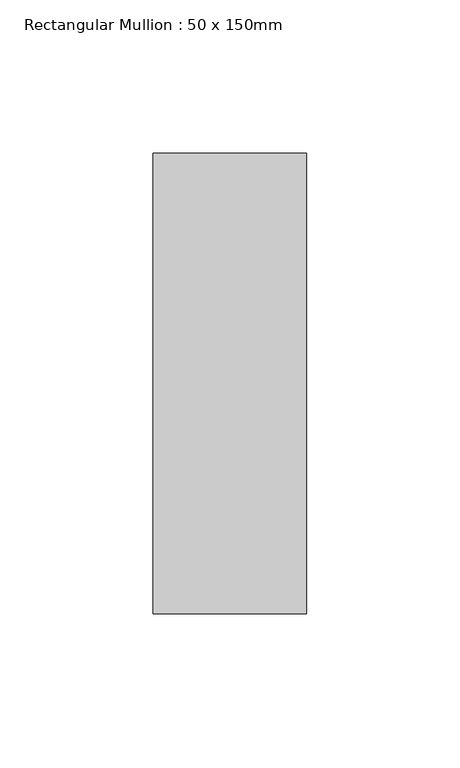
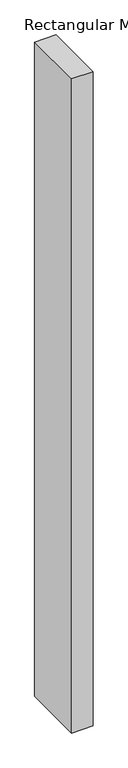
"""IFC4 building model written with IfcOpenShell, lengths in millimetres: member geometry, Rectangular Mullion : 50 x 150mm."""

from ifc_helpers import new_model, si_unit, frame, origin, place, context, project, spatial, polyline, outline, extrude, source, transform, mapped, element, save


def rectangular_mullion_50_x_150mm_d897cc90(model_context):
    return source(origin(), model_context, "Body", "SweptSolid", [
        extrude(outline(polyline([(0.0, 75.0), (0.0, -75.0), (-50.0, -75.0), (-50.0, 75.0), (0.0, 75.0)])), frame((0.0, 0.0, -1615.0), z_axis=(0.0, 0.0, 1.0), x_axis=(1.0, 0.0, 0.0)), (0.0, 0.0, 1.0), 1615.0),
    ])


if __name__ == "__main__":
    model = new_model("IFC4")
    model_context = context("Model", 3, world=origin())
    ifc_project = project(units=[si_unit("LENGTHUNIT", "METRE", prefix="MILLI")], contexts=[model_context])
    site = spatial("IfcSite", under=ifc_project)
    building = spatial("IfcBuilding", under=site)
    placement = place(None, origin())
    rectangular_mullion_50_x_150mm_shape = rectangular_mullion_50_x_150mm_d897cc90(model_context)
    element("IfcMember", 1, ObjectType="Rectangular Mullion : 50 x 150mm", at=placement, inside=building, context=model_context, shape_type="MappedRepresentation", body=[
        mapped(rectangular_mullion_50_x_150mm_shape, transform((0.0, 0.0, 0.0), x_axis=(1.0, 0.0, 0.0), y_axis=(0.0, 1.0, 0.0), z_axis=(0.0, 0.0, 1.0))),
    ])
    save(model, "model.ifc")

# Revit data of these elements
# Type "Rectangular Mullion : 50 x 150mm"
#   built-in parameter 1007304 = 0.492126 (stored number, unit not read)
#   built-in parameter 1007301 = 0.082021 (stored number, unit not read)
#   built-in parameter 1007300 = 0.082021 (stored number, unit not read)
# Element 1 (IfcMember, "Rectangular Mullion : 50 x 150mm")
#   Materials on its faces: "Metal - Aluminium"
# Materials
#   "Metal - Aluminium": class "Metal", colour RGB 247 247 247, transparency 0
